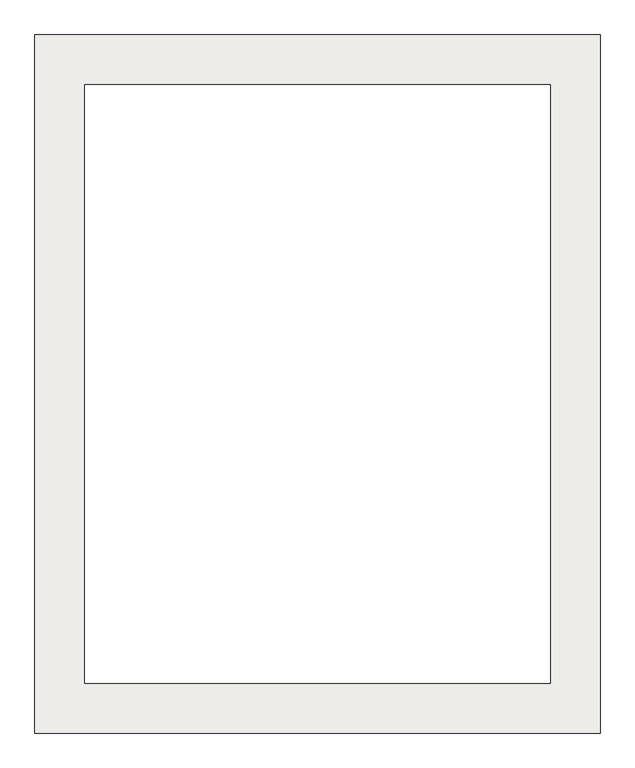
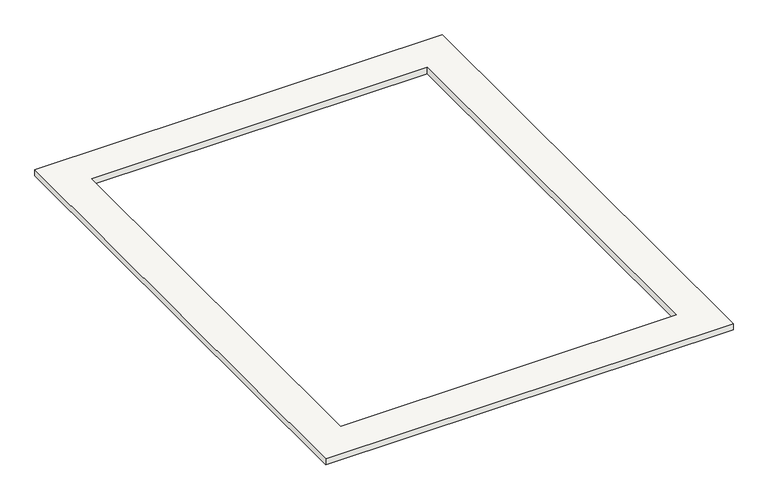
"""IFC4 building model written with IfcOpenShell, lengths in millimetres: slab geometry, Holzdecke."""

from ifc_helpers import new_model, si_unit, origin, origin_with_axes, place, context, project, spatial, polyline, outline, extrude, source, transform, mapped, element, save


def slab_b5571979(model_context):
    return source(origin(), model_context, "Body", "SweptSolid", [
        extrude(outline(polyline([(17000.0, 21002.8619019), (17000.0, 0.0), (0.0, 0.0), (0.0, 21002.8619019), (17000.0, 21002.8619019)]), holes=[polyline([(15500.0, 1500.0), (15500.0, 19502.8619019), (1500.0, 19502.8619019), (1500.0, 1500.0), (15500.0, 1500.0)])]), origin_with_axes(), (0.0, 0.0, 1.0), 270.0),
    ])


if __name__ == "__main__":
    model = new_model("IFC4")
    model_context = context("Model", 3, world=origin())
    ifc_project = project(units=[si_unit("LENGTHUNIT", "METRE", prefix="MILLI")], contexts=[model_context])
    site = spatial("IfcSite", under=ifc_project)
    building = spatial("IfcBuilding", under=site)
    placement = place(None, origin())
    slab_shape = slab_b5571979(model_context)
    element("IfcSlab", 1, ObjectType="Holzdecke", at=placement, inside=building, context=model_context, shape_type="MappedRepresentation", body=[
        mapped(slab_shape, transform((0.0, 0.0, 0.0), x_axis=(1.0, 0.0, 0.0), y_axis=(0.0, 1.0, 0.0), z_axis=(0.0, 0.0, 1.0))),
    ])
    save(model, "model.ifc")

# Revit data of these elements
# Element 1 (IfcSlab, "Holzdecke")
#   Materials on its faces: "holzschalung"
# Materials
#   "holzschalung": class "Unassigned", colour RGB 128 128 128, transparency 0
